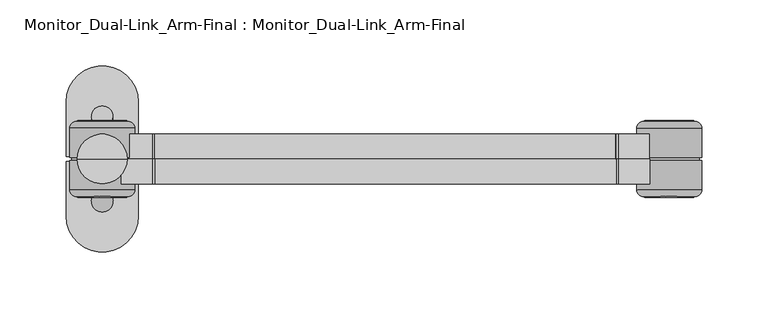
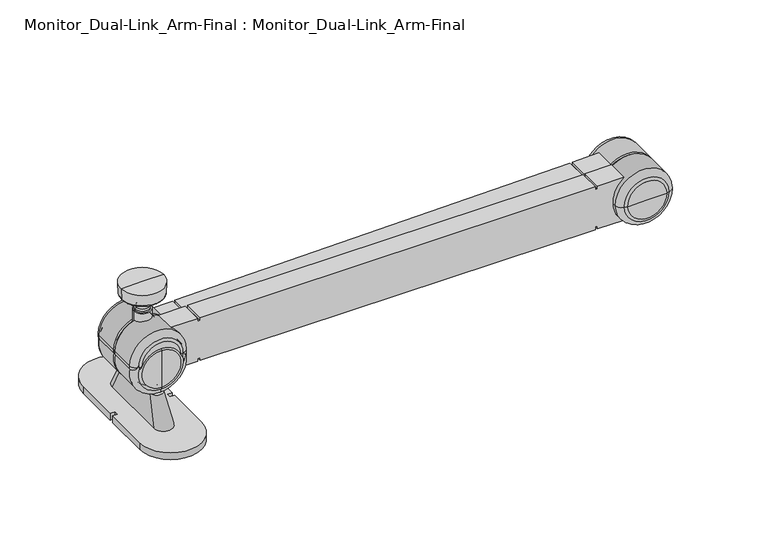
"""IFC4 building model written with IfcOpenShell, lengths in millimetres: proxy geometry, Monitor_Dual-Link_Arm-Final : Monitor_Dual-Link_Arm-Final."""

import ifcopenshell
import ifcopenshell.guid

model = None  # the IFC model being written
_history = None  # IfcOwnerHistory: only IFC2X3 demands one
_inside = {}  # id of a spatial element -> (the spatial element, [elements in it])
_under = {}  # id of a project, library or spatial element -> (it, [spatial elements below it])
_declared = {}  # id of a project -> (the project, [libraries it declares])
_typed = {}  # id of a type object -> (the type object, [elements of that type])
_made_of = {}  # id of a material, layer set ... -> (it, [elements and type objects made of it])


def new_model(schema):
    """Start an empty IFC model of exactly this schema.

    Asked for "IFC4X3", IfcOpenShell would pick the latest addendum, in which some entities
    have other attributes; the version numbers below select the first issue.
    IFC2X3 requires an IfcOwnerHistory on every rooted entity: one is made here for all.
    """
    global model, _history
    if schema == "IFC4X3":
        model = ifcopenshell.file(schema_version=(4, 3, 0, 0))
    else:
        model = ifcopenshell.file(schema=schema)
    _inside.clear()
    _under.clear()
    _declared.clear()
    _typed.clear()
    _made_of.clear()
    _history = None
    if model.schema == "IFC2X3":
        org = make("IfcOrganization", Name="unknown")
        user = make(
            "IfcPersonAndOrganization",
            ThePerson=make("IfcPerson", FamilyName="unknown"),
            TheOrganization=org,
        )
        app = make(
            "IfcApplication",
            ApplicationDeveloper=org,
            Version="unknown",
            ApplicationFullName="unknown",
            ApplicationIdentifier="unknown",
        )
        _history = make(
            "IfcOwnerHistory",
            OwningUser=user,
            OwningApplication=app,
            ChangeAction="ADDED",
            CreationDate=0,
        )
    return model


def make(cls, **values):
    """One entity of the class cls with the attributes given. An attribute that is None is left unset."""
    return model.create_entity(
        cls, **{name: value for name, value in values.items() if value is not None}
    )


def rooted(cls, **values):
    """An entity with a GlobalId (a new one), such as an element, a storey or a relation."""
    return make(cls, GlobalId=ifcopenshell.guid.new(), OwnerHistory=_history, **values)


def si_unit(unit_type, name, prefix=None):
    """IfcSIUnit, for example si_unit("LENGTHUNIT", "METRE", prefix="MILLI")."""
    return make("IfcSIUnit", UnitType=unit_type, Prefix=prefix, Name=name)


def assignment(units):
    """IfcUnitAssignment: the units of a project."""
    return None if units is None else make("IfcUnitAssignment", Units=units)


def point(xyz):
    """IfcCartesianPoint."""
    return None if xyz is None else make("IfcCartesianPoint", Coordinates=xyz)


def direction(xyz):
    """IfcDirection."""
    return None if xyz is None else make("IfcDirection", DirectionRatios=xyz)


def frame(location, z_axis=None, x_axis=None):
    """IfcAxis2Placement3D, a coordinate frame: its origin and axes. An axis left out is left unset."""
    return make(
        "IfcAxis2Placement3D",
        Location=point(location),
        Axis=direction(z_axis),
        RefDirection=direction(x_axis),
    )


def frame_2d(location, x_axis=None):
    """IfcAxis2Placement2D, a coordinate frame in the plane: its origin and x axis."""
    return make(
        "IfcAxis2Placement2D", Location=point(location), RefDirection=direction(x_axis)
    )


def origin():
    """The frame at (0, 0, 0) with its axes left unset."""
    return frame((0.0, 0.0, 0.0))


def origin_with_axes():
    """The frame at (0, 0, 0) with the z axis (0, 0, 1) and the x axis (1, 0, 0) written out."""
    return frame((0.0, 0.0, 0.0), z_axis=(0.0, 0.0, 1.0), x_axis=(1.0, 0.0, 0.0))


def place(relative_to, where):
    """IfcLocalPlacement: puts the frame where relative to a parent placement (None: the world)."""
    return make(
        "IfcLocalPlacement", PlacementRelTo=relative_to, RelativePlacement=where
    )


def context(
    kind, dimensions, precision=None, world=None, true_north=None, identifier=None
):
    """IfcGeometricRepresentationContext, for example the 3D "Model" context."""
    return make(
        "IfcGeometricRepresentationContext",
        ContextIdentifier=identifier,
        ContextType=kind,
        CoordinateSpaceDimension=dimensions,
        Precision=precision,
        WorldCoordinateSystem=world,
        TrueNorth=true_north,
    )


def project(units=None, contexts=None):
    """IfcProject with its units and contexts."""
    return rooted(
        "IfcProject",
        Name="project",
        RepresentationContexts=contexts,
        UnitsInContext=assignment(units),
    )


def spatial(cls, under=None, at=None, **own):
    """A site, building, storey or space (cls), placed at a placement, below another one or the project."""
    s = rooted(cls, ObjectPlacement=at, **own)
    if under is not None:
        _under.setdefault(under.id(), (under, []))[1].append(s)
    return s


def polyline(points):
    """IfcPolyline through the points."""
    return make("IfcPolyline", Points=[point(p) for p in points])


def circle_curve(where, radius):
    """IfcCircle in the frame where."""
    return make("IfcCircle", Position=where, Radius=radius)


def ellipse_curve(where, semi_axis1, semi_axis2):
    """IfcEllipse in the frame where."""
    return make(
        "IfcEllipse", Position=where, SemiAxis1=semi_axis1, SemiAxis2=semi_axis2
    )


def trimmed(basis, trim1, trim2, sense, master):
    """IfcTrimmedCurve: the piece of a basis curve between two trims."""
    return make(
        "IfcTrimmedCurve",
        BasisCurve=basis,
        Trim1=trim1,
        Trim2=trim2,
        SenseAgreement=sense,
        MasterRepresentation=master,
    )


def segment(curve, same_sense, transition):
    """IfcCompositeCurveSegment."""
    return make(
        "IfcCompositeCurveSegment",
        Transition=transition,
        SameSense=same_sense,
        ParentCurve=curve,
    )


def composite_curve(segments, self_intersect=None):
    """IfcCompositeCurve: segments joined end to end."""
    return make("IfcCompositeCurve", Segments=segments, SelfIntersect=self_intersect)


def outline(outer, holes=None, kind="AREA"):
    """IfcArbitraryClosedProfileDef: a profile drawn as a closed curve; with holes, ...WithVoids."""
    if holes is None:
        return make("IfcArbitraryClosedProfileDef", ProfileType=kind, OuterCurve=outer)
    return make(
        "IfcArbitraryProfileDefWithVoids",
        ProfileType=kind,
        OuterCurve=outer,
        InnerCurves=holes,
    )


def extrude(swept, where, along, depth):
    """IfcExtrudedAreaSolid: the profile swept, set in the frame where, extruded along a direction by depth."""
    return make(
        "IfcExtrudedAreaSolid",
        SweptArea=swept,
        Position=where,
        ExtrudedDirection=direction(along),
        Depth=depth,
    )


def shape(context_of_items, identifier, shape_type, items):
    """IfcShapeRepresentation: the items that make up one representation, for example the "Body"."""
    return make(
        "IfcShapeRepresentation",
        ContextOfItems=context_of_items,
        RepresentationIdentifier=identifier,
        RepresentationType=shape_type,
        Items=items,
    )


def source(mapping_origin, context_of_items, identifier, shape_type, items):
    """IfcRepresentationMap: a shape defined once, which mapped items show again and again."""
    return make(
        "IfcRepresentationMap",
        MappingOrigin=mapping_origin,
        MappedRepresentation=shape(context_of_items, identifier, shape_type, items),
    )


def transform(
    local_origin,
    x_axis=None,
    y_axis=None,
    z_axis=None,
    scale=None,
    scale2=None,
    scale3=None,
    uniform=True,
):
    """IfcCartesianTransformationOperator3D, or its non-uniform kind. x_axis, y_axis, z_axis: its Axis1, 2, 3."""
    if uniform:
        return make(
            "IfcCartesianTransformationOperator3D",
            Axis1=direction(x_axis),
            Axis2=direction(y_axis),
            LocalOrigin=point(local_origin),
            Scale=scale,
            Axis3=direction(z_axis),
        )
    return make(
        "IfcCartesianTransformationOperator3DnonUniform",
        Axis1=direction(x_axis),
        Axis2=direction(y_axis),
        LocalOrigin=point(local_origin),
        Scale=scale,
        Axis3=direction(z_axis),
        Scale2=scale2,
        Scale3=scale3,
    )


def mapped(mapping_source, mapping_target):
    """IfcMappedItem: shows the shape of a source again, moved by a transform."""
    return make(
        "IfcMappedItem", MappingSource=mapping_source, MappingTarget=mapping_target
    )


def made_of(thing, what):
    """Note that an element or type object is made of a material, layer set ...; save() writes the relation."""
    if what is not None:
        _made_of.setdefault(what.id(), (what, []))[1].append(thing)
    return thing


def element(
    cls,
    number,
    at=None,
    inside=None,
    cuts=None,
    type_object=None,
    material=None,
    context=None,
    identifier="Body",
    shape_type=None,
    held_by="IfcProductDefinitionShape",
    body=None,
    shapes=None,
    **own,
):
    """One element of the class cls, such as IfcWall. Its Tag is "e" and its number.

    at: its placement. inside: the storey or other place that contains it. cuts: it is an
    opening in that element (IfcRelVoidsElement). A single representation is given by context,
    identifier, shape_type and body (its items); several are given by shapes. held_by: the class
    of the entity that holds the representations. save() writes the other relations.
    """
    e = rooted(cls, Tag="e%d" % number, ObjectPlacement=at, **own)
    if body is not None:
        shapes = [shape(context, identifier, shape_type, body)]
    if shapes is not None:
        e.Representation = make(held_by, Representations=shapes)
    if inside is not None:
        _inside.setdefault(inside.id(), (inside, []))[1].append(e)
    if cuts is not None:
        rooted(
            "IfcRelVoidsElement", RelatingBuildingElement=cuts, RelatedOpeningElement=e
        )
    if type_object is not None:
        _typed.setdefault(type_object.id(), (type_object, []))[1].append(e)
    return made_of(e, material)


def aggregate(whole, parts):
    """IfcRelAggregates: a whole, such as a stair, and the parts it consists of."""
    return rooted("IfcRelAggregates", RelatingObject=whole, RelatedObjects=parts)


def save(model, path):
    """Write the relations noted so far, then the file.

    IfcRelAggregates (storeys below a building ...), IfcRelContainedInSpatialStructure (elements
    in a storey), IfcRelDefinesByType, IfcRelAssociatesMaterial and IfcRelDeclares: one each for
    every whole, place, type object, material and project.
    """
    for whole, parts in _under.values():
        aggregate(whole, parts)
    for where, things in _inside.values():
        rooted(
            "IfcRelContainedInSpatialStructure",
            RelatedElements=things,
            RelatingStructure=where,
        )
    for kind, things in _typed.values():
        rooted("IfcRelDefinesByType", RelatedObjects=things, RelatingType=kind)
    for what, things in _made_of.values():
        rooted("IfcRelAssociatesMaterial", RelatedObjects=things, RelatingMaterial=what)
    for by, libraries in _declared.values():
        rooted("IfcRelDeclares", RelatingContext=by, RelatedDefinitions=libraries)
    model.write(path)


def plane_surface(at):
    """IfcPlane: the flat surface through the origin of the frame at, square to its z axis."""
    return make("IfcPlane", Position=at)


def cylinder_surface(at, radius):
    """IfcCylindricalSurface: all points at the distance radius from the z axis of the frame at."""
    return make("IfcCylindricalSurface", Position=at, Radius=radius)


def revolved_surface(curve, axis_point, axis_direction):
    """IfcSurfaceOfRevolution: the curve turned about the line through axis_point along axis_direction."""
    return make(
        "IfcSurfaceOfRevolution",
        SweptCurve=make("IfcArbitraryOpenProfileDef", ProfileType="CURVE", Curve=curve),
        AxisPosition=make("IfcAxis1Placement", Location=point(axis_point), Axis=direction(axis_direction)),
    )


def spline_surface(u_degree, v_degree, points, u_multiplicities, v_multiplicities, u_knots, v_knots, weights=None):
    """IfcBSplineSurfaceWithKnots; with weights, IfcRationalBSplineSurfaceWithKnots. points: one row for each step in u."""
    own = dict(
        UDegree=u_degree,
        VDegree=v_degree,
        ControlPointsList=[[point(p) for p in row] for row in points],
        SurfaceForm="UNSPECIFIED",
        UClosed=False,
        VClosed=False,
        SelfIntersect=False,
        UMultiplicities=u_multiplicities,
        VMultiplicities=v_multiplicities,
        UKnots=u_knots,
        VKnots=v_knots,
        KnotSpec="UNSPECIFIED",
    )
    if weights is None:
        return make("IfcBSplineSurfaceWithKnots", **own)
    return make("IfcRationalBSplineSurfaceWithKnots", WeightsData=weights, **own)


def advanced_brep(points, edges, surfaces, faces):
    """IfcAdvancedBrep: a solid bounded by faces that lie on surfaces and meet in shared edges.

    An edge is (start, end): straight between two places in points (the first is 0);
    or (start, end, curve); or (start, end, curve, False) where it runs against its curve.
    A face is (place in surfaces, loops), or (place, loops, False) where it looks against
    its surface's normal. A loop lists edges by number (the first is 1), with a minus sign
    where the edge is run from its end to its start. The first loop is the outer one.
    """
    corners = [point(p) for p in points]
    vertices = [make("IfcVertexPoint", VertexGeometry=c) for c in corners]
    made = []
    for start, end, *more in edges:
        made.append(
            make(
                "IfcEdgeCurve",
                EdgeStart=vertices[start],
                EdgeEnd=vertices[end],
                EdgeGeometry=more[0] if more else make("IfcPolyline", Points=[corners[start], corners[end]]),
                SameSense=more[1] if len(more) > 1 else True,
            )
        )
    hull = []
    for where, loops, *sense in faces:
        bounds = []
        for j, loop in enumerate(loops):
            ring = [make("IfcOrientedEdge", EdgeElement=made[abs(k) - 1], Orientation=k > 0) for k in loop]
            bounds.append(
                make(
                    "IfcFaceOuterBound" if j == 0 else "IfcFaceBound",
                    Bound=make("IfcEdgeLoop", EdgeList=ring),
                    Orientation=True,
                )
            )
        hull.append(make("IfcAdvancedFace", Bounds=bounds, FaceSurface=surfaces[where], SameSense=sense[0] if sense else True))
    return make("IfcAdvancedBrep", Outer=make("IfcClosedShell", CfsFaces=hull))


def monitor_dual_link_arm_final_monitor_dual_link_arm_final_3c1dcffe(model_context):
    return source(origin(), model_context, "Body", "SolidModel", [
        advanced_brep(
        [(14.2594417, 0.0, 109.9159285), (-14.390005, 0.0, 109.9159285), (-17.2631298, 0.0, 109.9159285), (17.1325665, 0.0, 109.9159285), (10.4651235, 0.0, 108.0417995), (-10.5956869, 0.0, 108.0417995), (8.3225601, 0.0, 106.5415605), (-8.4531234, 0.0, 106.5415605), (2.4235287, 0.0, 106.4080746), (-2.554092, 0.0, 106.4080746), (2.4235287, 0.0, 104.7329669), (-2.554092, 0.0, 104.7329669), (3.4032162, 0.0, 104.7329669), (-3.5337796, 0.0, 104.7329669), (3.8485234, 0.0, 101.4790226), (-3.9790867, 0.0, 101.4790226), (5.3589975, 0.0, 98.9342238), (-5.4895609, 0.0, 98.9342238), (6.0692452, 0.0, 97.4110928), (-6.1998085, 0.0, 97.4110928), (6.0692452, 0.0, 96.0678917), (-6.1998085, 0.0, 96.0678917), (7.4106237, 0.0, 96.0678917), (-7.541187, 0.0, 96.0678917), (7.4106237, 0.0, 84.2810725), (-7.541187, 0.0, 84.2810725), (-0.0652817, 0.0, 84.2810725), (18.758255, 0.0, 120.873411), (-18.8888183, 0.0, 120.873411), (-0.0652817, 0.0, 120.873411), (18.3332726, 0.0, 111.1466342), (-18.4638359, 0.0, 111.1466342)],
        [
            (0, 1, circle_curve(frame((-0.0652817, 0.0, 109.9159285), z_axis=(0.0, 0.0, 1.0), x_axis=(-1.0, 0.0, 0.0)), 14.3247233)),
            (1, 2),
            (2, 3, circle_curve(frame((-0.0652817, 0.0, 109.9159285), z_axis=(0.0, 0.0, -1.0), x_axis=(-1.0, 0.0, 0.0)), 17.1978481)),
            (3, 0),
            (1, 0, circle_curve(frame((-0.0652817, 0.0, 109.9159285), z_axis=(0.0, 0.0, 1.0), x_axis=(-1.0, 0.0, 0.0)), 14.3247233)),
            (3, 2, circle_curve(frame((-0.0652817, 0.0, 109.9159285), z_axis=(0.0, 0.0, -1.0), x_axis=(-1.0, 0.0, 0.0)), 17.1978481)),
            (4, 5, circle_curve(frame((-0.0652817, 0.0, 108.0417995), z_axis=(0.0, 0.0, 1.0), x_axis=(-1.0, 0.0, 0.0)), 10.5304052)),
            (5, 1, circle_curve(frame((-14.6071665, 0.0, 104.6982593), z_axis=(0.0, -1.0, 0.0), x_axis=(0.0, 0.0, 1.0)), 5.2221864)),
            (0, 4, circle_curve(frame((14.4766032, 0.0, 104.6982593), z_axis=(0.0, -1.0, 0.0), x_axis=(0.0, 0.0, 1.0)), 5.2221864)),
            (5, 4, circle_curve(frame((-0.0652817, 0.0, 108.0417995), z_axis=(0.0, 0.0, 1.0), x_axis=(-1.0, 0.0, 0.0)), 10.5304052)),
            (6, 7, circle_curve(frame((-0.0652817, 0.0, 106.5415605), z_axis=(0.0, 0.0, 1.0), x_axis=(-1.0, 0.0, 0.0)), 8.3878417)),
            (7, 5, circle_curve(frame((-6.7614159, 0.0, 111.2376375), z_axis=(0.0, 1.0, 0.0), x_axis=(0.0, 0.0, 1.0)), 4.9914942)),
            (4, 6, circle_curve(frame((6.6308526, 0.0, 111.2376375), z_axis=(0.0, 1.0, 0.0), x_axis=(0.0, 0.0, 1.0)), 4.9914942)),
            (7, 6, circle_curve(frame((-0.0652817, 0.0, 106.5415605), z_axis=(0.0, 0.0, 1.0), x_axis=(-1.0, 0.0, 0.0)), 8.3878417)),
            (8, 9, circle_curve(frame((-0.0652817, 0.0, 106.4080746), z_axis=(0.0, 0.0, 1.0), x_axis=(-1.0, 0.0, 0.0)), 2.4888103)),
            (9, 7, circle_curve(frame((-1.755604, 0.0, 272.1072465), z_axis=(0.0, 1.0, 0.0), x_axis=(0.0, 0.0, 1.0)), 165.7010958)),
            (6, 8, circle_curve(frame((1.6250407, 0.0, 272.1072465), z_axis=(0.0, 1.0, 0.0), x_axis=(0.0, 0.0, 1.0)), 165.7010958)),
            (9, 8, circle_curve(frame((-0.0652817, 0.0, 106.4080746), z_axis=(0.0, 0.0, 1.0), x_axis=(-1.0, 0.0, 0.0)), 2.4888103)),
            (10, 11, circle_curve(frame((-0.0652817, 0.0, 104.7329669), z_axis=(0.0, 0.0, 1.0), x_axis=(-1.0, 0.0, 0.0)), 2.4888103)),
            (11, 9),
            (8, 10),
            (11, 10, circle_curve(frame((-0.0652817, 0.0, 104.7329669), z_axis=(0.0, 0.0, 1.0), x_axis=(-1.0, 0.0, 0.0)), 2.4888103)),
            (12, 13, circle_curve(frame((-0.0652817, 0.0, 104.7329669), z_axis=(0.0, 0.0, 1.0), x_axis=(-1.0, 0.0, 0.0)), 3.4684979)),
            (13, 11),
            (10, 12),
            (13, 12, circle_curve(frame((-0.0652817, 0.0, 104.7329669), z_axis=(0.0, 0.0, 1.0), x_axis=(-1.0, 0.0, 0.0)), 3.4684979)),
            (14, 15, circle_curve(frame((-0.0652817, 0.0, 101.4790226), z_axis=(0.0, 0.0, 1.0), x_axis=(-1.0, 0.0, 0.0)), 3.9138051)),
            (15, 13),
            (12, 14),
            (15, 14, circle_curve(frame((-0.0652817, 0.0, 101.4790226), z_axis=(0.0, 0.0, 1.0), x_axis=(-1.0, 0.0, 0.0)), 3.9138051)),
            (16, 17, circle_curve(frame((-0.0652817, 0.0, 98.9342238), z_axis=(0.0, 0.0, 1.0), x_axis=(-1.0, 0.0, 0.0)), 5.4242792)),
            (17, 15),
            (14, 16),
            (17, 16, circle_curve(frame((-0.0652817, 0.0, 98.9342238), z_axis=(0.0, 0.0, 1.0), x_axis=(-1.0, 0.0, 0.0)), 5.4242792)),
            (18, 19, circle_curve(frame((-0.0652817, 0.0, 97.4110928), z_axis=(0.0, 0.0, 1.0), x_axis=(-1.0, 0.0, 0.0)), 6.1345269)),
            (19, 17),
            (16, 18),
            (19, 18, circle_curve(frame((-0.0652817, 0.0, 97.4110928), z_axis=(0.0, 0.0, 1.0), x_axis=(-1.0, 0.0, 0.0)), 6.1345269)),
            (20, 21, circle_curve(frame((-0.0652817, 0.0, 96.0678917), z_axis=(0.0, 0.0, 1.0), x_axis=(-1.0, 0.0, 0.0)), 6.1345269)),
            (21, 19),
            (18, 20),
            (21, 20, circle_curve(frame((-0.0652817, 0.0, 96.0678917), z_axis=(0.0, 0.0, 1.0), x_axis=(-1.0, 0.0, 0.0)), 6.1345269)),
            (22, 23, circle_curve(frame((-0.0652817, 0.0, 96.0678917), z_axis=(0.0, 0.0, 1.0), x_axis=(-1.0, 0.0, 0.0)), 7.4759054)),
            (23, 21),
            (20, 22),
            (23, 22, circle_curve(frame((-0.0652817, 0.0, 96.0678917), z_axis=(0.0, 0.0, 1.0), x_axis=(-1.0, 0.0, 0.0)), 7.4759054)),
            (24, 25, circle_curve(frame((-0.0652817, 0.0, 84.2810725), z_axis=(0.0, 0.0, 1.0), x_axis=(-1.0, 0.0, 0.0)), 7.4759054)),
            (25, 23),
            (22, 24),
            (25, 24, circle_curve(frame((-0.0652817, 0.0, 84.2810725), z_axis=(0.0, 0.0, 1.0), x_axis=(-1.0, 0.0, 0.0)), 7.4759054)),
            (26, 25),
            (24, 26),
            (27, 28, circle_curve(frame((-0.0652817, 0.0, 120.873411), z_axis=(0.0, 0.0, 1.0), x_axis=(-1.0, 0.0, 0.0)), 18.8235367)),
            (28, 29),
            (29, 27),
            (28, 27, circle_curve(frame((-0.0652817, 0.0, 120.873411), z_axis=(0.0, 0.0, 1.0), x_axis=(-1.0, 0.0, 0.0)), 18.8235367)),
            (30, 31, circle_curve(frame((-0.0652817, 0.0, 111.1466342), z_axis=(0.0, 0.0, 1.0), x_axis=(-1.0, 0.0, 0.0)), 18.3985543)),
            (31, 28),
            (27, 30),
            (31, 30, circle_curve(frame((-0.0652817, 0.0, 111.1466342), z_axis=(0.0, 0.0, 1.0), x_axis=(-1.0, 0.0, 0.0)), 18.3985543)),
            (2, 31, circle_curve(frame((-17.1750383, 0.0, 111.2029444), z_axis=(0.0, 1.0, 0.0), x_axis=(0.0, 0.0, 1.0)), 1.2900272)),
            (30, 3, circle_curve(frame((17.044475, 0.0, 111.2029444), z_axis=(0.0, 1.0, 0.0), x_axis=(0.0, 0.0, 1.0)), 1.2900272)),
        ],
        [
            plane_surface(frame((-0.0652817, 0.0, 109.9159285), z_axis=(0.0, 0.0, -1.0), x_axis=(-1.0, 0.0, 0.0))),
            revolved_surface(trimmed(ellipse_curve(frame((-14.6071665, 0.0, 104.6982593), z_axis=(0.0, 1.0, 0.0), x_axis=(0.0, 0.0, 1.0)), 5.2221864, 5.2221864), [point((-14.390005, 0.0, 109.9159285))], [point((-10.5956869, 0.0, 108.0417995))], True, "CARTESIAN"), (-0.0652817, 0.0, 120.873411), (0.0, 0.0, -1.0)),
            revolved_surface(trimmed(ellipse_curve(frame((-6.7614159, 0.0, 111.2376375), z_axis=(0.0, -1.0, 0.0), x_axis=(0.0, 0.0, 1.0)), 4.9914942, 4.9914942), [point((-10.5956869, 0.0, 108.0417995))], [point((-8.4531234, 0.0, 106.5415605))], True, "CARTESIAN"), (-0.0652817, 0.0, 120.873411), (0.0, 0.0, -1.0)),
            revolved_surface(trimmed(ellipse_curve(frame((-1.755604, 0.0, 272.1072465), z_axis=(0.0, -1.0, 0.0), x_axis=(0.0, 0.0, 1.0)), 165.7010958, 165.7010958), [point((-8.4531234, 0.0, 106.5415605))], [point((-2.554092, 0.0, 106.4080746))], True, "CARTESIAN"), (-0.0652817, 0.0, 120.873411), (0.0, 0.0, -1.0)),
            cylinder_surface(frame((-0.0652817, 0.0, 120.873411), z_axis=(0.0, 0.0, -1.0), x_axis=(-1.0, 0.0, 0.0)), 2.4888103),
            plane_surface(frame((-0.0652817, 0.0, 104.7329669), z_axis=(0.0, 0.0, 1.0), x_axis=(-1.0, 0.0, 0.0))),
            revolved_surface(polyline([(-3.5337796, 0.0, 104.7329669), (-3.9790867, 0.0, 101.4790226)]), (-0.0652817, 0.0, 120.873411), (0.0, 0.0, -1.0)),
            revolved_surface(polyline([(-3.9790867, 0.0, 101.4790226), (-5.4895609, 0.0, 98.9342238)]), (-0.0652817, 0.0, 120.873411), (0.0, 0.0, -1.0)),
            revolved_surface(polyline([(-5.4895609, 0.0, 98.9342238), (-6.1998085, 0.0, 97.4110928)]), (-0.0652817, 0.0, 120.873411), (0.0, 0.0, -1.0)),
            cylinder_surface(frame((-0.0652817, 0.0, 120.873411), z_axis=(0.0, 0.0, -1.0), x_axis=(-1.0, 0.0, 0.0)), 6.1345269),
            plane_surface(frame((-0.0652817, 0.0, 96.0678917), z_axis=(0.0, 0.0, 1.0), x_axis=(-1.0, 0.0, 0.0))),
            cylinder_surface(frame((-0.0652817, 0.0, 120.873411), z_axis=(0.0, 0.0, -1.0), x_axis=(-1.0, 0.0, 0.0)), 7.4759054),
            plane_surface(frame((-0.0652817, 0.0, 84.2810725), z_axis=(0.0, 0.0, -1.0), x_axis=(-1.0, 0.0, 0.0))),
            plane_surface(frame((-0.0652817, 0.0, 120.873411), z_axis=(0.0, 0.0, 1.0), x_axis=(-1.0, 0.0, 0.0))),
            revolved_surface(polyline([(-18.8888183, 0.0, 120.873411), (-18.4638359, 0.0, 111.1466342)]), (-0.0652817, 0.0, 120.873411), (0.0, 0.0, -1.0)),
            revolved_surface(trimmed(ellipse_curve(frame((-17.1750383, 0.0, 111.2029444), z_axis=(0.0, -1.0, 0.0), x_axis=(0.0, 0.0, 1.0)), 1.2900272, 1.2900272), [point((-18.4638359, 0.0, 111.1466342))], [point((-17.2631298, 0.0, 109.9159285))], True, "CARTESIAN"), (-0.0652817, 0.0, 120.873411), (0.0, 0.0, -1.0)),
        ],
        [
            (0, [[1, 2, 3, 4]]),
            (0, [[5, -4, 6, -2]]),
            (1, [[7, 8, -1, 9]]),
            (1, [[10, -9, -5, -8]]),
            (2, [[11, 12, -7, 13]]),
            (2, [[14, -13, -10, -12]]),
            (3, [[15, 16, -11, 17]]),
            (3, [[18, -17, -14, -16]]),
            (4, [[19, 20, -15, 21]]),
            (4, [[22, -21, -18, -20]]),
            (5, [[23, 24, -19, 25]]),
            (5, [[26, -25, -22, -24]]),
            (6, [[27, 28, -23, 29]]),
            (6, [[30, -29, -26, -28]]),
            (7, [[31, 32, -27, 33]]),
            (7, [[34, -33, -30, -32]]),
            (8, [[35, 36, -31, 37]]),
            (8, [[38, -37, -34, -36]]),
            (9, [[39, 40, -35, 41]]),
            (9, [[42, -41, -38, -40]]),
            (10, [[43, 44, -39, 45]]),
            (10, [[46, -45, -42, -44]]),
            (11, [[47, 48, -43, 49]]),
            (11, [[50, -49, -46, -48]]),
            (12, [[51, -47, 52]]),
            (12, [[-52, -50, -51]]),
            (13, [[53, 54, 55]]),
            (13, [[56, -55, -54]]),
            (14, [[57, 58, -53, 59]]),
            (14, [[60, -59, -56, -58]]),
            (15, [[-3, 61, -57, 62]]),
            (15, [[-6, -62, -60, -61]]),
        ],
    ),
        extrude(outline(composite_curve([segment(polyline([(84.5121655, 413.9843004), (84.5121655, 390.5634677), (82.0815253, 390.5634677), (82.0815253, 388.5392194), (84.5121655, 388.5392194), (84.5121655, 39.9552173), (82.0815253, 39.9552173), (82.0815253, 37.9309689), (84.5121655, 37.9309689), (84.5121655, 14.5101363)]), True, "CONTINUOUS"), segment(trimmed(circle_curve(frame_2d((64.6305377, -0.0652817)), 24.6520168), [point((84.5121655, 14.5101363))], [point((64.6305377, 24.5867352))], True, "CARTESIAN"), True, "CONTINUOUS"), segment(trimmed(circle_curve(frame_2d((64.6305377, -0.0652817)), 24.6520168), [point((64.6305377, 24.5867352))], [point((44.7489099, 14.5101363))], True, "CARTESIAN"), True, "CONTINUOUS"), segment(polyline([(44.7489099, 14.5101363), (44.7489099, 37.9309689), (47.1795501, 37.9309689), (47.1795501, 39.9552173), (44.7489099, 39.9552173), (44.7489099, 388.5392194), (47.1795501, 388.5392194), (47.1795501, 390.5634677), (44.7489099, 390.5634677), (44.7489099, 413.9843004)]), True, "CONTINUOUS"), segment(trimmed(circle_curve(frame_2d((64.6305377, 428.5597183)), 24.6520168), [point((44.7489099, 413.9843004))], [point((64.6305377, 403.9077015))], True, "CARTESIAN"), True, "CONTINUOUS"), segment(trimmed(circle_curve(frame_2d((64.6305377, 428.5597183)), 24.6520168), [point((64.6305377, 403.9077015))], [point((84.5121655, 413.9843004))], True, "CARTESIAN"), True, "CONTINUOUS")], self_intersect=False)), frame((0.0, -19.05, 0.0), z_axis=(0.0, 1.0, 0.0), x_axis=(0.0, 0.0, 1.0)), (0.0, 0.0, 1.0), 19.05),
        extrude(outline(composite_curve([segment(polyline([(37.5257763, 14.9201803), (37.9345262, 38.3374458), (40.3647963, 38.2950253), (40.4001243, 40.3189654), (37.9698542, 40.3613859), (44.0534839, 388.892297), (46.483754, 388.8498764), (46.519082, 390.8738165), (44.0888119, 390.916237), (44.4975618, 414.3335025)]), True, "CONTINUOUS"), segment(trimmed(circle_curve(frame_2d((64.6305377, 428.5597183)), 24.6520168), [point((44.4975618, 414.3335025))], [point((64.2003007, 403.9114561))], True, "CARTESIAN"), True, "CONTINUOUS"), segment(trimmed(circle_curve(frame_2d((64.6305377, 428.5597183)), 24.6520168), [point((64.2003007, 403.9114561))], [point((84.2547614, 413.639538))], True, "CARTESIAN"), True, "CONTINUOUS"), segment(polyline([(84.2547614, 413.639538), (83.8460115, 390.2222725), (81.4157414, 390.264693), (81.3804134, 388.240753), (83.8106835, 388.1983325), (77.7270538, 39.6674214), (75.2967837, 39.7098419), (75.2614557, 37.6859019), (77.6917258, 37.6434813), (77.2829759, 14.2262158)]), True, "CONTINUOUS"), segment(trimmed(circle_curve(frame_2d((57.15, 0.0)), 24.6520168), [point((77.2829759, 14.2262158))], [point((57.580237, 24.6482622))], True, "CARTESIAN"), True, "CONTINUOUS"), segment(trimmed(circle_curve(frame_2d((57.15, 0.0)), 24.6520168), [point((57.580237, 24.6482622))], [point((37.5257763, 14.9201803))], True, "CARTESIAN"), True, "CONTINUOUS")], self_intersect=False)), frame((0.0, 0.0, 0.0), z_axis=(0.0, 1.0, 0.0), x_axis=(0.0, 0.0, 1.0)), (0.0, 0.0, 1.0), 19.05),
        advanced_brep(
        [(0.0, -29.2471299, 74.2044566), (0.0, -29.2471299, 40.0955434), (0.0, -29.2471299, 57.15), (0.0, -28.2791366, 76.8005348), (0.0, -28.2791366, 37.4994652), (0.0, -23.3656038, 81.8020168), (0.0, -23.3656038, 32.4979832), (0.0, -1.1824193, 81.8020168), (0.0, -1.1824193, 32.4979832), (0.0, -1.1824193, 79.9979466), (0.0, -1.1824193, 34.3020534), (0.0, 1.1824193, 79.9979466), (0.0, 1.1824193, 34.3020534), (0.0, 1.1824193, 81.8020168), (0.0, 1.1824193, 32.4979832), (0.0, 23.3656038, 81.8020168), (0.0, 23.3656038, 32.4979832), (0.0, 28.2791366, 76.8005348), (0.0, 28.2791366, 37.4994652), (0.0, 29.2471299, 74.2044566), (0.0, 29.2471299, 40.0955434), (0.0, 29.2471299, 57.15)],
        [
            (0, 1, circle_curve(frame((0.0, -29.2471299, 57.15), z_axis=(0.0, -1.0, 0.0), x_axis=(0.0, 0.0, -1.0)), 17.0544566)),
            (1, 2),
            (2, 0),
            (1, 0, circle_curve(frame((0.0, -29.2471299, 57.15), z_axis=(0.0, -1.0, 0.0), x_axis=(0.0, 0.0, -1.0)), 17.0544566)),
            (3, 4, circle_curve(frame((0.0, -28.2791366, 57.15), z_axis=(0.0, -1.0, 0.0), x_axis=(0.0, 0.0, -1.0)), 19.6505348)),
            (4, 1, circle_curve(frame((0.0, -25.5205933, 40.0065422), z_axis=(-1.0, 0.0, 0.0), x_axis=(0.0, 1.0, 0.0)), 3.7275992)),
            (0, 3, circle_curve(frame((0.0, -25.5205933, 74.2934578), z_axis=(-1.0, 0.0, 0.0), x_axis=(0.0, 1.0, 0.0)), 3.7275992)),
            (4, 3, circle_curve(frame((0.0, -28.2791366, 57.15), z_axis=(0.0, -1.0, 0.0), x_axis=(0.0, 0.0, -1.0)), 19.6505348)),
            (5, 6, circle_curve(frame((0.0, -23.3656038, 57.15), z_axis=(0.0, -1.0, 0.0), x_axis=(0.0, 0.0, -1.0)), 24.6520168)),
            (6, 4, circle_curve(frame((0.0, -23.2768674, 37.4994652), z_axis=(-1.0, 0.0, 0.0), x_axis=(0.0, 1.0, 0.0)), 5.0022691)),
            (3, 5, circle_curve(frame((0.0, -23.2768674, 76.8005348), z_axis=(-1.0, 0.0, 0.0), x_axis=(0.0, 1.0, 0.0)), 5.0022691)),
            (6, 5, circle_curve(frame((0.0, -23.3656038, 57.15), z_axis=(0.0, -1.0, 0.0), x_axis=(0.0, 0.0, -1.0)), 24.6520168)),
            (7, 8, circle_curve(frame((0.0, -1.1824193, 57.15), z_axis=(0.0, -1.0, 0.0), x_axis=(0.0, 0.0, -1.0)), 24.6520168)),
            (8, 6),
            (5, 7),
            (8, 7, circle_curve(frame((0.0, -1.1824193, 57.15), z_axis=(0.0, -1.0, 0.0), x_axis=(0.0, 0.0, -1.0)), 24.6520168)),
            (9, 10, circle_curve(frame((0.0, -1.1824193, 57.15), z_axis=(0.0, -1.0, 0.0), x_axis=(0.0, 0.0, -1.0)), 22.8479466)),
            (10, 8),
            (7, 9),
            (10, 9, circle_curve(frame((0.0, -1.1824193, 57.15), z_axis=(0.0, -1.0, 0.0), x_axis=(0.0, 0.0, -1.0)), 22.8479466)),
            (11, 12, circle_curve(frame((0.0, 1.1824193, 57.15), z_axis=(0.0, -1.0, 0.0), x_axis=(0.0, 0.0, -1.0)), 22.8479466)),
            (12, 10),
            (9, 11),
            (12, 11, circle_curve(frame((0.0, 1.1824193, 57.15), z_axis=(0.0, -1.0, 0.0), x_axis=(0.0, 0.0, -1.0)), 22.8479466)),
            (13, 14, circle_curve(frame((0.0, 1.1824193, 57.15), z_axis=(0.0, -1.0, 0.0), x_axis=(0.0, 0.0, -1.0)), 24.6520168)),
            (14, 12),
            (11, 13),
            (14, 13, circle_curve(frame((0.0, 1.1824193, 57.15), z_axis=(0.0, -1.0, 0.0), x_axis=(0.0, 0.0, -1.0)), 24.6520168)),
            (15, 16, circle_curve(frame((0.0, 23.3656038, 57.15), z_axis=(0.0, -1.0, 0.0), x_axis=(0.0, 0.0, -1.0)), 24.6520168)),
            (16, 14),
            (13, 15),
            (16, 15, circle_curve(frame((0.0, 23.3656038, 57.15), z_axis=(0.0, -1.0, 0.0), x_axis=(0.0, 0.0, -1.0)), 24.6520168)),
            (17, 18, circle_curve(frame((0.0, 28.2791366, 57.15), z_axis=(0.0, -1.0, 0.0), x_axis=(0.0, 0.0, -1.0)), 19.6505348)),
            (18, 16, circle_curve(frame((0.0, 23.2768674, 37.4994652), z_axis=(-1.0, 0.0, 0.0), x_axis=(0.0, 1.0, 0.0)), 5.0022691)),
            (15, 17, circle_curve(frame((0.0, 23.2768674, 76.8005348), z_axis=(-1.0, 0.0, 0.0), x_axis=(0.0, 1.0, 0.0)), 5.0022691)),
            (18, 17, circle_curve(frame((0.0, 28.2791366, 57.15), z_axis=(0.0, -1.0, 0.0), x_axis=(0.0, 0.0, -1.0)), 19.6505348)),
            (19, 20, circle_curve(frame((0.0, 29.2471299, 57.15), z_axis=(0.0, -1.0, 0.0), x_axis=(0.0, 0.0, -1.0)), 17.0544566)),
            (20, 18, circle_curve(frame((0.0, 25.5205933, 40.0065422), z_axis=(-1.0, 0.0, 0.0), x_axis=(0.0, 1.0, 0.0)), 3.7275992)),
            (17, 19, circle_curve(frame((0.0, 25.5205933, 74.2934578), z_axis=(-1.0, 0.0, 0.0), x_axis=(0.0, 1.0, 0.0)), 3.7275992)),
            (20, 19, circle_curve(frame((0.0, 29.2471299, 57.15), z_axis=(0.0, -1.0, 0.0), x_axis=(0.0, 0.0, -1.0)), 17.0544566)),
            (21, 20),
            (19, 21),
        ],
        [
            plane_surface(frame((0.0, -29.2471299, 57.15), z_axis=(0.0, -1.0, 0.0), x_axis=(0.0, 0.0, -1.0))),
            revolved_surface(trimmed(ellipse_curve(frame((0.0, -25.5205933, 40.0065422), z_axis=(1.0, 0.0, 0.0), x_axis=(0.0, 1.0, 0.0)), 3.7275992, 3.7275992), [point((0.0, -29.2471299, 40.0955434))], [point((0.0, -28.2791366, 37.4994652))], True, "CARTESIAN"), (0.0, 29.2471299, 57.15), (0.0, 1.0, 0.0)),
            revolved_surface(trimmed(ellipse_curve(frame((0.0, -23.2768674, 37.4994652), z_axis=(1.0, 0.0, 0.0), x_axis=(0.0, 1.0, 0.0)), 5.0022691, 5.0022691), [point((0.0, -28.2791366, 37.4994652))], [point((0.0, -23.3656038, 32.4979832))], True, "CARTESIAN"), (0.0, 29.2471299, 57.15), (0.0, 1.0, 0.0)),
            cylinder_surface(frame((0.0, 29.2471299, 57.15), z_axis=(0.0, 1.0, 0.0), x_axis=(0.0, 0.0, -1.0)), 24.6520168),
            plane_surface(frame((0.0, -1.1824193, 57.15), z_axis=(0.0, 1.0, 0.0), x_axis=(0.0, 0.0, -1.0))),
            cylinder_surface(frame((0.0, 29.2471299, 57.15), z_axis=(0.0, 1.0, 0.0), x_axis=(0.0, 0.0, -1.0)), 22.8479466),
            plane_surface(frame((0.0, 1.1824193, 57.15), z_axis=(0.0, -1.0, 0.0), x_axis=(0.0, 0.0, -1.0))),
            revolved_surface(trimmed(ellipse_curve(frame((0.0, 23.2768674, 37.4994652), z_axis=(1.0, 0.0, 0.0), x_axis=(0.0, 1.0, 0.0)), 5.0022691, 5.0022691), [point((0.0, 23.3656038, 32.4979832))], [point((0.0, 28.2791366, 37.4994652))], True, "CARTESIAN"), (0.0, 29.2471299, 57.15), (0.0, 1.0, 0.0)),
            revolved_surface(trimmed(ellipse_curve(frame((0.0, 25.5205933, 40.0065422), z_axis=(1.0, 0.0, 0.0), x_axis=(0.0, 1.0, 0.0)), 3.7275992, 3.7275992), [point((0.0, 28.2791366, 37.4994652))], [point((0.0, 29.2471299, 40.0955434))], True, "CARTESIAN"), (0.0, 29.2471299, 57.15), (0.0, 1.0, 0.0)),
            plane_surface(frame((0.0, 29.2471299, 57.15), z_axis=(0.0, 1.0, 0.0), x_axis=(0.0, 0.0, -1.0))),
        ],
        [
            (0, [[1, 2, 3]]),
            (0, [[4, -3, -2]]),
            (1, [[5, 6, -1, 7]]),
            (1, [[8, -7, -4, -6]]),
            (2, [[9, 10, -5, 11]]),
            (2, [[12, -11, -8, -10]]),
            (3, [[13, 14, -9, 15]]),
            (3, [[16, -15, -12, -14]]),
            (4, [[17, 18, -13, 19]]),
            (4, [[20, -19, -16, -18]]),
            (5, [[21, 22, -17, 23]]),
            (5, [[24, -23, -20, -22]]),
            (6, [[25, 26, -21, 27]]),
            (6, [[28, -27, -24, -26]]),
            (3, [[29, 30, -25, 31]]),
            (3, [[32, -31, -28, -30]]),
            (7, [[33, 34, -29, 35]]),
            (7, [[36, -35, -32, -34]]),
            (8, [[37, 38, -33, 39]]),
            (8, [[40, -39, -36, -38]]),
            (9, [[41, -37, 42]]),
            (9, [[-42, -40, -41]]),
        ],
    ),
        advanced_brep(
        [(-17.1197382, -29.2471299, 64.6305377), (16.9891749, -29.2471299, 64.6305377), (-0.0652817, -29.2471299, 64.6305377), (-19.7158165, -28.2791366, 64.6305377), (19.5852532, -28.2791366, 64.6305377), (-24.7172985, -23.3656038, 64.6305377), (24.5867352, -23.3656038, 64.6305377), (-24.7172985, -1.1824193, 64.6305377), (24.5867352, -1.1824193, 64.6305377), (-22.9132283, -1.1824193, 64.6305377), (22.782665, -1.1824193, 64.6305377), (-22.9132283, 1.1824193, 64.6305377), (22.782665, 1.1824193, 64.6305377), (-24.7172985, 1.1824193, 64.6305377), (24.5867352, 1.1824193, 64.6305377), (-24.7172985, 23.3656038, 64.6305377), (24.5867352, 23.3656038, 64.6305377), (-19.7158165, 28.2791366, 64.6305377), (19.5852532, 28.2791366, 64.6305377), (-17.1197382, 29.2471299, 64.6305377), (16.9891749, 29.2471299, 64.6305377), (-0.0652817, 29.2471299, 64.6305377)],
        [
            (0, 1, circle_curve(frame((-0.0652817, -29.2471299, 64.6305377), z_axis=(0.0, -1.0, 0.0), x_axis=(1.0, 0.0, 0.0)), 17.0544566)),
            (1, 2),
            (2, 0),
            (1, 0, circle_curve(frame((-0.0652817, -29.2471299, 64.6305377), z_axis=(0.0, -1.0, 0.0), x_axis=(1.0, 0.0, 0.0)), 17.0544566)),
            (3, 4, circle_curve(frame((-0.0652817, -28.2791366, 64.6305377), z_axis=(0.0, -1.0, 0.0), x_axis=(1.0, 0.0, 0.0)), 19.6505348)),
            (4, 1, circle_curve(frame((17.0781761, -25.5205933, 64.6305377), z_axis=(0.0, 0.0, -1.0), x_axis=(-1.0, 0.0, 0.0)), 3.7275992)),
            (0, 3, circle_curve(frame((-17.2087395, -25.5205933, 64.6305377), z_axis=(0.0, 0.0, -1.0), x_axis=(1.0, 0.0, 0.0)), 3.7275992)),
            (4, 3, circle_curve(frame((-0.0652817, -28.2791366, 64.6305377), z_axis=(0.0, -1.0, 0.0), x_axis=(1.0, 0.0, 0.0)), 19.6505348)),
            (5, 6, circle_curve(frame((-0.0652817, -23.3656038, 64.6305377), z_axis=(0.0, -1.0, 0.0), x_axis=(1.0, 0.0, 0.0)), 24.6520168)),
            (6, 4, circle_curve(frame((19.5852532, -23.2768674, 64.6305377), z_axis=(0.0, 0.0, -1.0), x_axis=(-1.0, 0.0, 0.0)), 5.0022691)),
            (3, 5, circle_curve(frame((-19.7158165, -23.2768674, 64.6305377), z_axis=(0.0, 0.0, -1.0), x_axis=(1.0, 0.0, 0.0)), 5.0022691)),
            (6, 5, circle_curve(frame((-0.0652817, -23.3656038, 64.6305377), z_axis=(0.0, -1.0, 0.0), x_axis=(1.0, 0.0, 0.0)), 24.6520168)),
            (7, 8, circle_curve(frame((-0.0652817, -1.1824193, 64.6305377), z_axis=(0.0, -1.0, 0.0), x_axis=(1.0, 0.0, 0.0)), 24.6520168)),
            (8, 6),
            (5, 7),
            (8, 7, circle_curve(frame((-0.0652817, -1.1824193, 64.6305377), z_axis=(0.0, -1.0, 0.0), x_axis=(1.0, 0.0, 0.0)), 24.6520168)),
            (9, 10, circle_curve(frame((-0.0652817, -1.1824193, 64.6305377), z_axis=(0.0, -1.0, 0.0), x_axis=(1.0, 0.0, 0.0)), 22.8479466)),
            (10, 8),
            (7, 9),
            (10, 9, circle_curve(frame((-0.0652817, -1.1824193, 64.6305377), z_axis=(0.0, -1.0, 0.0), x_axis=(1.0, 0.0, 0.0)), 22.8479466)),
            (11, 12, circle_curve(frame((-0.0652817, 1.1824193, 64.6305377), z_axis=(0.0, -1.0, 0.0), x_axis=(1.0, 0.0, 0.0)), 22.8479466)),
            (12, 10),
            (9, 11),
            (12, 11, circle_curve(frame((-0.0652817, 1.1824193, 64.6305377), z_axis=(0.0, -1.0, 0.0), x_axis=(1.0, 0.0, 0.0)), 22.8479466)),
            (13, 14, circle_curve(frame((-0.0652817, 1.1824193, 64.6305377), z_axis=(0.0, -1.0, 0.0), x_axis=(1.0, 0.0, 0.0)), 24.6520168)),
            (14, 12),
            (11, 13),
            (14, 13, circle_curve(frame((-0.0652817, 1.1824193, 64.6305377), z_axis=(0.0, -1.0, 0.0), x_axis=(1.0, 0.0, 0.0)), 24.6520168)),
            (15, 16, circle_curve(frame((-0.0652817, 23.3656038, 64.6305377), z_axis=(0.0, -1.0, 0.0), x_axis=(1.0, 0.0, 0.0)), 24.6520168)),
            (16, 14),
            (13, 15),
            (16, 15, circle_curve(frame((-0.0652817, 23.3656038, 64.6305377), z_axis=(0.0, -1.0, 0.0), x_axis=(1.0, 0.0, 0.0)), 24.6520168)),
            (17, 18, circle_curve(frame((-0.0652817, 28.2791366, 64.6305377), z_axis=(0.0, -1.0, 0.0), x_axis=(1.0, 0.0, 0.0)), 19.6505348)),
            (18, 16, circle_curve(frame((19.5852532, 23.2768674, 64.6305377), z_axis=(0.0, 0.0, -1.0), x_axis=(-1.0, 0.0, 0.0)), 5.0022691)),
            (15, 17, circle_curve(frame((-19.7158165, 23.2768674, 64.6305377), z_axis=(0.0, 0.0, -1.0), x_axis=(1.0, 0.0, 0.0)), 5.0022691)),
            (18, 17, circle_curve(frame((-0.0652817, 28.2791366, 64.6305377), z_axis=(0.0, -1.0, 0.0), x_axis=(1.0, 0.0, 0.0)), 19.6505348)),
            (19, 20, circle_curve(frame((-0.0652817, 29.2471299, 64.6305377), z_axis=(0.0, -1.0, 0.0), x_axis=(1.0, 0.0, 0.0)), 17.0544566)),
            (20, 18, circle_curve(frame((17.0781761, 25.5205933, 64.6305377), z_axis=(0.0, 0.0, -1.0), x_axis=(-1.0, 0.0, 0.0)), 3.7275992)),
            (17, 19, circle_curve(frame((-17.2087395, 25.5205933, 64.6305377), z_axis=(0.0, 0.0, -1.0), x_axis=(1.0, 0.0, 0.0)), 3.7275992)),
            (20, 19, circle_curve(frame((-0.0652817, 29.2471299, 64.6305377), z_axis=(0.0, -1.0, 0.0), x_axis=(1.0, 0.0, 0.0)), 17.0544566)),
            (21, 20),
            (19, 21),
        ],
        [
            plane_surface(frame((-0.0652817, -29.2471299, 64.6305377), z_axis=(0.0, -1.0, 0.0), x_axis=(1.0, 0.0, 0.0))),
            revolved_surface(trimmed(ellipse_curve(frame((17.0781761, -25.5205933, 64.6305377), z_axis=(0.0, 0.0, 1.0), x_axis=(-1.0, 0.0, 0.0)), 3.7275992, 3.7275992), [point((16.9891749, -29.2471299, 64.6305377))], [point((19.5852532, -28.2791366, 64.6305377))], True, "CARTESIAN"), (-0.0652817, 29.2471299, 64.6305377), (0.0, 1.0, 0.0)),
            revolved_surface(trimmed(ellipse_curve(frame((19.5852532, -23.2768674, 64.6305377), z_axis=(0.0, 0.0, 1.0), x_axis=(-1.0, 0.0, 0.0)), 5.0022691, 5.0022691), [point((19.5852532, -28.2791366, 64.6305377))], [point((24.5867352, -23.3656038, 64.6305377))], True, "CARTESIAN"), (-0.0652817, 29.2471299, 64.6305377), (0.0, 1.0, 0.0)),
            cylinder_surface(frame((-0.0652817, 29.2471299, 64.6305377), z_axis=(0.0, 1.0, 0.0), x_axis=(1.0, 0.0, 0.0)), 24.6520168),
            plane_surface(frame((-0.0652817, -1.1824193, 64.6305377), z_axis=(0.0, 1.0, 0.0), x_axis=(1.0, 0.0, 0.0))),
            cylinder_surface(frame((-0.0652817, 29.2471299, 64.6305377), z_axis=(0.0, 1.0, 0.0), x_axis=(1.0, 0.0, 0.0)), 22.8479466),
            plane_surface(frame((-0.0652817, 1.1824193, 64.6305377), z_axis=(0.0, -1.0, 0.0), x_axis=(1.0, 0.0, 0.0))),
            revolved_surface(trimmed(ellipse_curve(frame((19.5852532, 23.2768674, 64.6305377), z_axis=(0.0, 0.0, 1.0), x_axis=(-1.0, 0.0, 0.0)), 5.0022691, 5.0022691), [point((24.5867352, 23.3656038, 64.6305377))], [point((19.5852532, 28.2791366, 64.6305377))], True, "CARTESIAN"), (-0.0652817, 29.2471299, 64.6305377), (0.0, 1.0, 0.0)),
            revolved_surface(trimmed(ellipse_curve(frame((17.0781761, 25.5205933, 64.6305377), z_axis=(0.0, 0.0, 1.0), x_axis=(-1.0, 0.0, 0.0)), 3.7275992, 3.7275992), [point((19.5852532, 28.2791366, 64.6305377))], [point((16.9891749, 29.2471299, 64.6305377))], True, "CARTESIAN"), (-0.0652817, 29.2471299, 64.6305377), (0.0, 1.0, 0.0)),
            plane_surface(frame((-0.0652817, 29.2471299, 64.6305377), z_axis=(0.0, 1.0, 0.0), x_axis=(1.0, 0.0, 0.0))),
        ],
        [
            (0, [[1, 2, 3]]),
            (0, [[4, -3, -2]]),
            (1, [[5, 6, -1, 7]]),
            (1, [[8, -7, -4, -6]]),
            (2, [[9, 10, -5, 11]]),
            (2, [[12, -11, -8, -10]]),
            (3, [[13, 14, -9, 15]]),
            (3, [[16, -15, -12, -14]]),
            (4, [[17, 18, -13, 19]]),
            (4, [[20, -19, -16, -18]]),
            (5, [[21, 22, -17, 23]]),
            (5, [[24, -23, -20, -22]]),
            (6, [[25, 26, -21, 27]]),
            (6, [[28, -27, -24, -26]]),
            (3, [[29, 30, -25, 31]]),
            (3, [[32, -31, -28, -30]]),
            (7, [[33, 34, -29, 35]]),
            (7, [[36, -35, -32, -34]]),
            (8, [[37, 38, -33, 39]]),
            (8, [[40, -39, -36, -38]]),
            (9, [[41, -37, 42]]),
            (9, [[-42, -40, -41]]),
        ],
    ),
        advanced_brep(
        [(445.6115774, -29.2471299, 64.928179), (411.5078592, -29.2471299, 64.3328964), (428.5597183, -29.2471299, 64.6305377), (448.2072603, -28.2791366, 64.9734868), (408.9121764, -28.2791366, 64.2875886), (453.2079805, -23.3656038, 65.0607747), (403.9114561, -23.3656038, 64.2003007), (451.4041851, -1.1824193, 65.0292894), (405.7152516, -1.1824193, 64.2317861), (403.9114561, -1.1824193, 64.2003007), (453.2079805, -1.1824193, 65.0607747), (451.4041851, 1.1824193, 65.0292894), (405.7152516, 1.1824193, 64.2317861), (453.2079805, 1.1824193, 65.0607747), (403.9114561, 1.1824193, 64.2003007), (448.2072603, 28.2791366, 64.9734868), (408.9121764, 28.2791366, 64.2875886), (403.9114561, 23.3656038, 64.2003007), (453.2079805, 23.3656038, 65.0607747), (445.6115774, 29.2471299, 64.928179), (411.5078592, 29.2471299, 64.3328964), (428.5597183, 29.2471299, 64.6305377)],
        [
            (0, 1, circle_curve(frame((428.5597183, -29.2471299, 64.6305377), z_axis=(0.0, -1.0, 0.0), x_axis=(-0.9998476951563913, 0.0, -0.01745240643728023)), 17.0544566)),
            (1, 2),
            (2, 0),
            (1, 0, circle_curve(frame((428.5597183, -29.2471299, 64.6305377), z_axis=(0.0, -1.0, 0.0), x_axis=(-0.9998476951563913, 0.0, -0.01745240643728023)), 17.0544566)),
            (3, 4, circle_curve(frame((428.5597183, -28.2791366, 64.6305377), z_axis=(0.0, -1.0, 0.0), x_axis=(-0.9998476951563913, 0.0, -0.01745240643728023)), 19.6505348)),
            (4, 1, circle_curve(frame((411.4188716, -25.5205933, 64.3313431), z_axis=(-0.017452406437280243, 0.0, 0.9998476951563913), x_axis=(0.9998476951563913, 0.0, 0.017452406437280243)), 3.7275992)),
            (0, 3, circle_curve(frame((445.7005651, -25.5205933, 64.9297323), z_axis=(-0.017452406437283473, 0.0, 0.9998476951563912), x_axis=(-0.9998476951563912, 0.0, -0.017452406437283473)), 3.7275992)),
            (4, 3, circle_curve(frame((428.5597183, -28.2791366, 64.6305377), z_axis=(0.0, -1.0, 0.0), x_axis=(-0.9998476951563913, 0.0, -0.01745240643728023)), 19.6505348)),
            (5, 6, circle_curve(frame((428.5597183, -23.3656038, 64.6305377), z_axis=(0.0, -1.0, 0.0), x_axis=(-0.9998476951563913, 0.0, -0.01745240643728023)), 24.6520168)),
            (6, 4, circle_curve(frame((408.9121764, -23.2768674, 64.2875886), z_axis=(-0.017452406437280243, 0.0, 0.9998476951563913), x_axis=(0.9998476951563913, 0.0, 0.017452406437280243)), 5.0022691)),
            (3, 5, circle_curve(frame((448.2072603, -23.2768674, 64.9734868), z_axis=(-0.017452406437283473, 0.0, 0.9998476951563912), x_axis=(-0.9998476951563912, 0.0, -0.017452406437283473)), 5.0022691)),
            (6, 5, circle_curve(frame((428.5597183, -23.3656038, 64.6305377), z_axis=(0.0, -1.0, 0.0), x_axis=(-0.9998476951563913, 0.0, -0.01745240643728023)), 24.6520168)),
            (7, 8, circle_curve(frame((428.5597183, -1.1824193, 64.6305377), z_axis=(0.0, -1.0, 0.0), x_axis=(-0.9998476951563913, 0.0, -0.01745240643728023)), 22.8479466)),
            (8, 9),
            (9, 10, circle_curve(frame((428.5597183, -1.1824193, 64.6305377), z_axis=(0.0, 1.0, 0.0), x_axis=(-0.9998476951563913, 0.0, -0.01745240643728023)), 24.6520168)),
            (10, 7),
            (8, 7, circle_curve(frame((428.5597183, -1.1824193, 64.6305377), z_axis=(0.0, -1.0, 0.0), x_axis=(-0.9998476951563913, 0.0, -0.01745240643728023)), 22.8479466)),
            (10, 9, circle_curve(frame((428.5597183, -1.1824193, 64.6305377), z_axis=(0.0, 1.0, 0.0), x_axis=(-0.9998476951563913, 0.0, -0.01745240643728023)), 24.6520168)),
            (11, 12, circle_curve(frame((428.5597183, 1.1824193, 64.6305377), z_axis=(0.0, -1.0, 0.0), x_axis=(-0.9998476951563913, 0.0, -0.01745240643728023)), 22.8479466)),
            (12, 8),
            (7, 11),
            (12, 11, circle_curve(frame((428.5597183, 1.1824193, 64.6305377), z_axis=(0.0, -1.0, 0.0), x_axis=(-0.9998476951563913, 0.0, -0.01745240643728023)), 22.8479466)),
            (13, 14, circle_curve(frame((428.5597183, 1.1824193, 64.6305377), z_axis=(0.0, -1.0, 0.0), x_axis=(-0.9998476951563913, 0.0, -0.01745240643728023)), 24.6520168)),
            (14, 12),
            (11, 13),
            (14, 13, circle_curve(frame((428.5597183, 1.1824193, 64.6305377), z_axis=(0.0, -1.0, 0.0), x_axis=(-0.9998476951563913, 0.0, -0.01745240643728023)), 24.6520168)),
            (15, 16, circle_curve(frame((428.5597183, 28.2791366, 64.6305377), z_axis=(0.0, -1.0, 0.0), x_axis=(-0.9998476951563913, 0.0, -0.01745240643728023)), 19.6505348)),
            (16, 17, circle_curve(frame((408.9121764, 23.2768674, 64.2875886), z_axis=(-0.017452406437280243, 0.0, 0.9998476951563913), x_axis=(0.9998476951563913, 0.0, 0.017452406437280243)), 5.0022691)),
            (17, 18, circle_curve(frame((428.5597183, 23.3656038, 64.6305377), z_axis=(0.0, 1.0, 0.0), x_axis=(-0.9998476951563913, 0.0, -0.01745240643728023)), 24.6520168)),
            (18, 15, circle_curve(frame((448.2072603, 23.2768674, 64.9734868), z_axis=(-0.017452406437283473, 0.0, 0.9998476951563912), x_axis=(-0.9998476951563912, 0.0, -0.017452406437283473)), 5.0022691)),
            (16, 15, circle_curve(frame((428.5597183, 28.2791366, 64.6305377), z_axis=(0.0, -1.0, 0.0), x_axis=(-0.9998476951563913, 0.0, -0.01745240643728023)), 19.6505348)),
            (18, 17, circle_curve(frame((428.5597183, 23.3656038, 64.6305377), z_axis=(0.0, 1.0, 0.0), x_axis=(-0.9998476951563913, 0.0, -0.01745240643728023)), 24.6520168)),
            (19, 20, circle_curve(frame((428.5597183, 29.2471299, 64.6305377), z_axis=(0.0, -1.0, 0.0), x_axis=(-0.9998476951563913, 0.0, -0.01745240643728023)), 17.0544566)),
            (20, 16, circle_curve(frame((411.4188716, 25.5205933, 64.3313431), z_axis=(-0.017452406437280243, 0.0, 0.9998476951563913), x_axis=(0.9998476951563913, 0.0, 0.017452406437280243)), 3.7275992)),
            (15, 19, circle_curve(frame((445.7005651, 25.5205933, 64.9297323), z_axis=(-0.017452406437283473, 0.0, 0.9998476951563912), x_axis=(-0.9998476951563912, 0.0, -0.017452406437283473)), 3.7275992)),
            (20, 19, circle_curve(frame((428.5597183, 29.2471299, 64.6305377), z_axis=(0.0, -1.0, 0.0), x_axis=(-0.9998476951563913, 0.0, -0.01745240643728023)), 17.0544566)),
            (21, 20),
            (19, 21),
            (9, 6),
            (5, 10),
            (17, 14),
            (13, 18),
        ],
        [
            plane_surface(frame((428.5597183, -29.2471299, 64.6305377), z_axis=(0.0, -1.0, 0.0), x_axis=(-0.9998476951563913, 0.0, -0.01745240643728023))),
            revolved_surface(trimmed(ellipse_curve(frame((411.4188716, -25.5205933, 64.3313431), z_axis=(0.017452406437280243, 0.0, -0.9998476951563913), x_axis=(0.9998476951563913, 0.0, 0.017452406437280243)), 3.7275992, 3.7275992), [point((411.5078592, -29.2471299, 64.3328964))], [point((408.9121764, -28.2791366, 64.2875886))], True, "CARTESIAN"), (428.5597183, 29.2471299, 64.6305377), (0.0, 1.0, 0.0)),
            revolved_surface(trimmed(ellipse_curve(frame((408.9121764, -23.2768674, 64.2875886), z_axis=(0.017452406437280243, 0.0, -0.9998476951563913), x_axis=(0.9998476951563913, 0.0, 0.017452406437280243)), 5.0022691, 5.0022691), [point((408.9121764, -28.2791366, 64.2875886))], [point((403.9114561, -23.3656038, 64.2003007))], True, "CARTESIAN"), (428.5597183, 29.2471299, 64.6305377), (0.0, 1.0, 0.0)),
            plane_surface(frame((428.5597183, -1.1824193, 64.6305377), z_axis=(0.0, 1.0, 0.0), x_axis=(-0.9998476951563913, 0.0, -0.01745240643728023))),
            cylinder_surface(frame((428.5597183, 29.2471299, 64.6305377), z_axis=(0.0, 1.0, 0.0), x_axis=(-0.9998476951563913, 0.0, -0.01745240643728023)), 22.8479466),
            plane_surface(frame((428.5597183, 1.1824193, 64.6305377), z_axis=(0.0, -1.0, 0.0), x_axis=(-0.9998476951563913, 0.0, -0.01745240643728023))),
            revolved_surface(trimmed(ellipse_curve(frame((408.9121764, 23.2768674, 64.2875886), z_axis=(0.017452406437280243, 0.0, -0.9998476951563913), x_axis=(0.9998476951563913, 0.0, 0.017452406437280243)), 5.0022691, 5.0022691), [point((403.9114561, 23.3656038, 64.2003007))], [point((408.9121764, 28.2791366, 64.2875886))], True, "CARTESIAN"), (428.5597183, 29.2471299, 64.6305377), (0.0, 1.0, 0.0)),
            revolved_surface(trimmed(ellipse_curve(frame((411.4188716, 25.5205933, 64.3313431), z_axis=(0.017452406437280243, 0.0, -0.9998476951563913), x_axis=(0.9998476951563913, 0.0, 0.017452406437280243)), 3.7275992, 3.7275992), [point((408.9121764, 28.2791366, 64.2875886))], [point((411.5078592, 29.2471299, 64.3328964))], True, "CARTESIAN"), (428.5597183, 29.2471299, 64.6305377), (0.0, 1.0, 0.0)),
            plane_surface(frame((428.5597183, 29.2471299, 64.6305377), z_axis=(0.0, 1.0, 0.0), x_axis=(-0.9998476951563913, 0.0, -0.01745240643728023))),
            cylinder_surface(frame((428.5597183, 29.2471299, 64.6305377), z_axis=(0.0, 1.0, 0.0), x_axis=(-0.9998476951563913, 0.0, -0.01745240643728023)), 24.6520168),
        ],
        [
            (0, [[1, 2, 3]]),
            (0, [[4, -3, -2]]),
            (1, [[5, 6, -1, 7]]),
            (1, [[8, -7, -4, -6]]),
            (2, [[9, 10, -5, 11]]),
            (2, [[12, -11, -8, -10]]),
            (3, [[13, 14, 15, 16]]),
            (3, [[17, -16, 18, -14]]),
            (4, [[19, 20, -13, 21]]),
            (4, [[22, -21, -17, -20]]),
            (5, [[23, 24, -19, 25]]),
            (5, [[26, -25, -22, -24]]),
            (6, [[27, 28, 29, 30]]),
            (6, [[31, -30, 32, -28]]),
            (7, [[33, 34, -27, 35]]),
            (7, [[36, -35, -31, -34]]),
            (8, [[37, -33, 38]]),
            (8, [[-38, -36, -37]]),
            (9, [[-15, 39, -9, 40]]),
            (9, [[-18, -40, -12, -39]]),
            (9, [[-29, 41, -23, 42]]),
            (9, [[-32, -42, -26, -41]]),
        ],
    ),
        advanced_brep(
        [(-5.5651166, -21.6115782, 31.75), (5.5651166, -21.6115782, 31.75), (5.5651166, 21.6115782, 31.75), (-5.5651166, 21.6115782, 31.75), (-8.2217789, -31.9284627, 6.35), (-8.2217789, 31.9284627, 6.35), (8.2217789, 31.9284627, 6.35), (8.2217789, -31.9284627, 6.35)],
        [
            (0, 1, circle_curve(frame((0.0, -21.6115782, 31.75), z_axis=(0.0, 0.0, 1.0), x_axis=(-1.0, 0.0, 0.0)), 5.5651166)),
            (1, 2),
            (2, 3, circle_curve(frame((0.0, 21.6115782, 31.75), z_axis=(0.0, 0.0, 1.0), x_axis=(-1.0, 0.0, 0.0)), 5.5651166)),
            (3, 0),
            (4, 5),
            (5, 6, circle_curve(frame((0.0, 31.9284627, 6.35), z_axis=(0.0, 0.0, -1.0), x_axis=(-1.0, 0.0, 0.0)), 8.2217789)),
            (6, 7),
            (7, 4, circle_curve(frame((0.0, -31.9284627, 6.35), z_axis=(0.0, 0.0, -1.0), x_axis=(-1.0, 0.0, 0.0)), 8.2217789)),
            (7, 1),
            (0, 4),
            (6, 2),
            (5, 3),
        ],
        [
            plane_surface(frame((0.0, 0.0, 31.75), z_axis=(0.0, 0.0, 1.0), x_axis=(0.0, -1.0, 0.0))),
            plane_surface(frame((0.0, 0.0, 6.35), z_axis=(0.0, 0.0, -1.0), x_axis=(0.0, -1.0, 0.0))),
            spline_surface(2, 1, [[(-8.2217789, -31.9284627, 6.35), (-5.5651166, -21.6115782, 31.75)], [(-8.2217789, -40.1502416, 6.35), (-5.5651166, -27.1766948, 31.75)], [(0.0, -40.1502416, 6.35), (0.0, -27.1766948, 31.75)], [(8.2217789, -40.1502416, 6.35), (5.5651166, -27.1766948, 31.75)], [(8.2217789, -31.9284627, 6.35), (5.5651166, -21.6115782, 31.75)]], [3, 2, 3], [2, 2], [0.0, 1.0, 2.0], [0.0, 1.0], weights=[[1.0, 1.0], [0.7071067811865476, 0.7071067811865476], [1.0, 1.0], [0.7071067811865476, 0.7071067811865476], [1.0, 1.0]]),
            plane_surface(frame((8.2217789, 0.0, 6.35), z_axis=(0.9945746253614987, 0.0, 0.1040255477612814), x_axis=(0.0, 1.0, 0.0))),
            spline_surface(2, 1, [[(8.2217789, 31.9284627, 6.35), (5.5651166, 21.6115782, 31.75)], [(8.2217789, 40.1502416, 6.35), (5.5651166, 27.1766948, 31.75)], [(0.0, 40.1502416, 6.35), (0.0, 27.1766948, 31.75)], [(-8.2217789, 40.1502416, 6.35), (-5.5651166, 27.1766948, 31.75)], [(-8.2217789, 31.9284627, 6.35), (-5.5651166, 21.6115782, 31.75)]], [3, 2, 3], [2, 2], [0.0, 1.0, 2.0], [0.0, 1.0], weights=[[1.0, 1.0], [0.7071067811865476, 0.7071067811865476], [1.0, 1.0], [0.7071067811865476, 0.7071067811865476], [1.0, 1.0]]),
            plane_surface(frame((-8.2217789, 0.0, 6.35), z_axis=(-0.9945746253615921, 0.0, 0.10402554776038764), x_axis=(0.0, -1.0, 0.0))),
        ],
        [
            (0, [[1, 2, 3, 4]]),
            (1, [[5, 6, 7, 8]]),
            (2, [[-8, 9, -1, 10]]),
            (3, [[-7, 11, -2, -9]]),
            (4, [[-6, 12, -3, -11]]),
            (5, [[-5, -10, -4, -12]]),
        ],
    ),
        extrude(outline(composite_curve([segment(polyline([(-23.0598856, -1.9848539), (-23.0598856, 1.9848539), (-27.2717789, 1.9848539), (-27.2717789, 43.2142987)]), True, "CONTINUOUS"), segment(trimmed(circle_curve(frame_2d((0.0, 43.2142987)), 27.2717789), [point((-27.2717789, 43.2142987))], [point((27.2717789, 43.2142987))], False, "CARTESIAN"), True, "CONTINUOUS"), segment(polyline([(27.2717789, 43.2142987), (27.2717789, 1.9848539), (23.0598856, 1.9848539), (23.0598856, -1.9848539), (27.2717789, -1.9848539), (27.2717789, -43.2142987)]), True, "CONTINUOUS"), segment(trimmed(circle_curve(frame_2d((0.0, -43.2142987)), 27.2717789), [point((27.2717789, -43.2142987))], [point((-27.2717789, -43.2142987))], False, "CARTESIAN"), True, "CONTINUOUS"), segment(polyline([(-27.2717789, -43.2142987), (-27.2717789, -1.9848539), (-23.0598856, -1.9848539)]), True, "CONTINUOUS")], self_intersect=False)), origin_with_axes(), (0.0, 0.0, 1.0), 6.35),
    ])


if __name__ == "__main__":
    model = new_model("IFC4")
    model_context = context("Model", 3, world=origin())
    ifc_project = project(units=[si_unit("LENGTHUNIT", "METRE", prefix="MILLI")], contexts=[model_context])
    site = spatial("IfcSite", under=ifc_project)
    building = spatial("IfcBuilding", under=site)
    placement = place(None, origin())
    monitor_dual_link_arm_final_monitor_dual_link_arm_final_shape = monitor_dual_link_arm_final_monitor_dual_link_arm_final_3c1dcffe(model_context)
    element("IfcBuildingElementProxy", 1, Name="Monitor_Dual-Link_Arm-Final : Monitor_Dual-Link_Arm-Final", ObjectType="Monitor_Dual-Link_Arm-Final : Monitor_Dual-Link_Arm-Final", at=placement, inside=building, context=model_context, shape_type="MappedRepresentation", body=[
        mapped(monitor_dual_link_arm_final_monitor_dual_link_arm_final_shape, transform((0.0, 0.0, 0.0), x_axis=(1.0, 0.0, 0.0), y_axis=(0.0, 1.0, 0.0), z_axis=(0.0, 0.0, 1.0))),
    ])
    save(model, "model.ifc")
